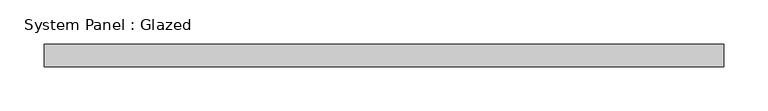
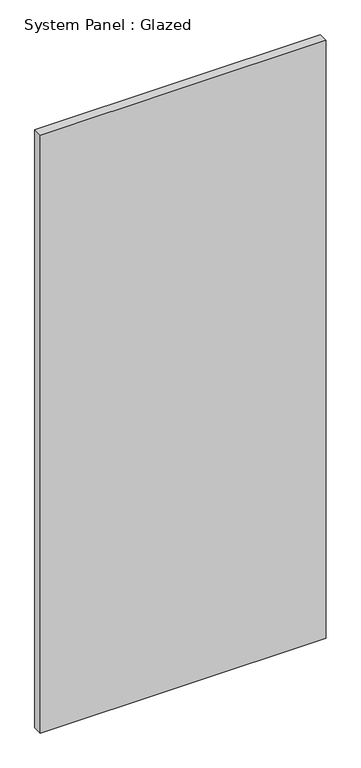
"""IFC4 building model written with IfcOpenShell, lengths in millimetres: plate geometry, System Panel : Glazed."""

from ifc_helpers import new_model, si_unit, origin, origin_with_axes, place, context, project, spatial, polyline, outline, extrude, source, transform, mapped, element, save


def system_panel_glazed_22d54c0a(model_context):
    return source(origin(), model_context, "Body", "SweptSolid", [
        extrude(outline(polyline([(384.9166667, 19.05), (-384.9166667, 19.05), (-384.9166667, 44.45), (384.9166667, 44.45), (384.9166667, 19.05)])), origin_with_axes(), (0.0, 0.0, 1.0), 1701.8),
    ])


if __name__ == "__main__":
    model = new_model("IFC4")
    model_context = context("Model", 3, world=origin())
    ifc_project = project(units=[si_unit("LENGTHUNIT", "METRE", prefix="MILLI")], contexts=[model_context])
    site = spatial("IfcSite", under=ifc_project)
    building = spatial("IfcBuilding", under=site)
    placement = place(None, origin())
    system_panel_glazed_shape = system_panel_glazed_22d54c0a(model_context)
    element("IfcPlate", 1, ObjectType="System Panel : Glazed", at=placement, inside=building, context=model_context, shape_type="MappedRepresentation", body=[
        mapped(system_panel_glazed_shape, transform((0.0, 0.0, 0.0), x_axis=(1.0, 0.0, 0.0), y_axis=(0.0, 1.0, 0.0), z_axis=(0.0, 0.0, 1.0))),
    ])
    save(model, "model.ifc")

# Revit data of these elements
# Element 1 (IfcPlate, "System Panel : Glazed")
#   Materials on its faces: "Glass"
# Materials
#   "Glass": class "Glass", colour RGB 0 128 192, transparency 0.75
